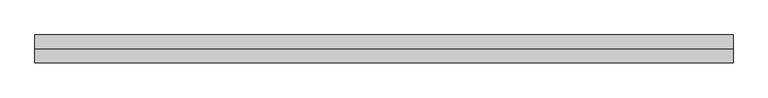
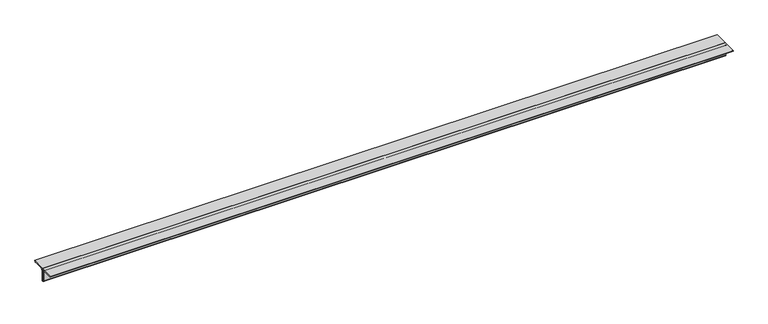
"""IFC4 building model written with IfcOpenShell, lengths in millimetres: member geometry, Steel Framing_2Ls_KS : H_SB_AR_S02_2Ls-100x100x10_VBR1."""

from ifc_helpers import new_model, si_unit, point, frame, frame_2d, origin, place, context, project, spatial, polyline, circle_curve, trimmed, segment, composite_curve, outline, extrude, source, transform, mapped, element, save


def member_4443a68e(model_context):
    return source(origin(), model_context, "Body", "SweptSolid", [
        extrude(outline(composite_curve([segment(polyline([(0.0, 28.2), (100.0, 28.2)]), True, "CONTINUOUS"), segment(trimmed(circle_curve(frame_2d((90.0, 28.2)), 10.0), [point((100.0, 28.2))], [point((90.0, 18.2))], False, "CARTESIAN"), True, "CONTINUOUS"), segment(polyline([(90.0, 18.2), (20.0, 18.2)]), True, "CONTINUOUS"), segment(trimmed(circle_curve(frame_2d((20.0, 8.2)), 10.0), [point((20.0, 18.2))], [point((10.0, 8.2))], True, "CARTESIAN"), True, "CONTINUOUS"), segment(polyline([(10.0, 8.2), (10.0, -61.8)]), True, "CONTINUOUS"), segment(trimmed(circle_curve(frame_2d((0.0, -61.8)), 10.0), [point((10.0, -61.8))], [point((0.0, -71.8))], False, "CARTESIAN"), True, "CONTINUOUS"), segment(polyline([(0.0, -71.8), (0.0, 28.2)]), True, "CONTINUOUS")], self_intersect=False)), frame((-2479.1576866, 0.0, 0.0), z_axis=(1.0, 0.0, 0.0), x_axis=(0.0, 1.0, 0.0)), (0.0, 0.0, 1.0), 4994.8078214),
        extrude(outline(composite_curve([segment(polyline([(0.0, 28.2), (0.0, -71.8)]), True, "CONTINUOUS"), segment(trimmed(circle_curve(frame_2d((0.0, -61.8)), 10.0), [point((0.0, -71.8))], [point((-10.0, -61.8))], False, "CARTESIAN"), True, "CONTINUOUS"), segment(polyline([(-10.0, -61.8), (-10.0, 8.2)]), True, "CONTINUOUS"), segment(trimmed(circle_curve(frame_2d((-20.0, 8.2)), 10.0), [point((-10.0, 8.2))], [point((-20.0, 18.2))], True, "CARTESIAN"), True, "CONTINUOUS"), segment(polyline([(-20.0, 18.2), (-90.0, 18.2)]), True, "CONTINUOUS"), segment(trimmed(circle_curve(frame_2d((-90.0, 28.2)), 10.0), [point((-90.0, 18.2))], [point((-100.0, 28.2))], False, "CARTESIAN"), True, "CONTINUOUS"), segment(polyline([(-100.0, 28.2), (0.0, 28.2)]), True, "CONTINUOUS")], self_intersect=False)), frame((-2479.1576866, 0.0, 0.0), z_axis=(1.0, 0.0, 0.0), x_axis=(0.0, 1.0, 0.0)), (0.0, 0.0, 1.0), 4994.8078214),
    ])


if __name__ == "__main__":
    model = new_model("IFC4")
    model_context = context("Model", 3, world=origin())
    ifc_project = project(units=[si_unit("LENGTHUNIT", "METRE", prefix="MILLI")], contexts=[model_context])
    site = spatial("IfcSite", under=ifc_project)
    building = spatial("IfcBuilding", under=site)
    placement = place(None, origin())
    member_shape = member_4443a68e(model_context)
    element("IfcMember", 1, ObjectType="Steel Framing_2Ls_KS : H_SB_AR_S02_2Ls-100x100x10_VBR1", at=placement, inside=building, context=model_context, shape_type="MappedRepresentation", body=[
        mapped(member_shape, transform((0.0, 0.0, 0.0), x_axis=(1.0, 0.0, 0.0), y_axis=(0.0, 1.0, 0.0), z_axis=(0.0, 0.0, 1.0))),
    ])
    save(model, "model.ifc")

# Revit data of these elements
# Type "Steel Framing_2Ls_KS : H_SB_AR_S02_2Ls-100x100x10_VBR1"
#   Type Comments = "MAIN"
#   Type Mark = "VBR1"
#   H_SectionID = "2Ls-100x100x10"
#   Assembly Code = "B10"
#   Legs = "LLBB"
#   H_Ratio for Additional Steel Plate = 0.2
#   W = 0
#   Perimeter = 0.80 m²/m
#   Nominal Weight = 29.80 kgf/m
#   Length [instance default] = 1524 mm
#   Space = 0 mm
#   b = 100 mm
#   d = 100 mm
#   t = 10 mm
#   y = 28.2 mm
#   A = 0.0038 m²
#   Structural Material [instance default] = Steel, 45-345
# Element 1 (IfcMember, "Steel Framing_2Ls_KS : H_SB_AR_S02_2Ls-100x100x10_VBR1")
#   Materials on its faces: "Steel, 45-345"
# Materials
#   "Steel, 45-345": class "Metal", colour RGB 189 187 185, transparency 0, Description = "Steel 345 MPa", Cost = 0
